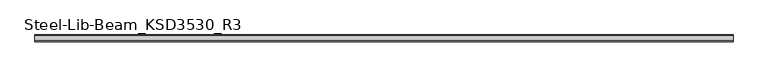
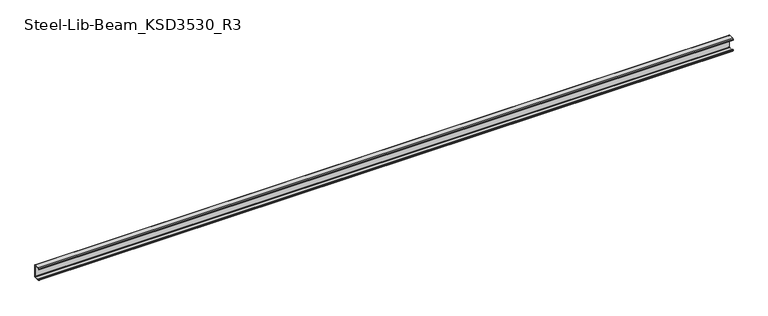
"""IFC4 building model written with IfcOpenShell, lengths in millimetres: beam geometry, Steel-Lib-Beam_KSD3530_R3 : BMS291_C-150×75x20x4.5."""

from ifc_helpers import new_model, si_unit, point, frame, frame_2d, origin, place, context, project, spatial, polyline, circle_curve, trimmed, segment, composite_curve, outline, extrude, source, transform, mapped, element, save


def steel_lib_beam_ksd3530_r3_927b0633(model_context):
    return source(origin(), model_context, "Body", "SweptSolid", [
        extrude(outline(composite_curve([segment(trimmed(circle_curve(frame_2d((-41.0, 66.0)), 9.0), [point((-50.0, 66.0))], [point((-41.0, 75.0))], False, "CARTESIAN"), True, "CONTINUOUS"), segment(polyline([(-41.0, 75.0), (16.0, 75.0)]), True, "CONTINUOUS"), segment(trimmed(circle_curve(frame_2d((16.0, 66.0)), 9.0), [point((16.0, 75.0))], [point((25.0, 66.0))], False, "CARTESIAN"), True, "CONTINUOUS"), segment(polyline([(25.0, 66.0), (25.0, -66.0)]), True, "CONTINUOUS"), segment(trimmed(circle_curve(frame_2d((16.0, -66.0)), 9.0), [point((25.0, -66.0))], [point((16.0, -75.0))], False, "CARTESIAN"), True, "CONTINUOUS"), segment(polyline([(16.0, -75.0), (-41.0, -75.0)]), True, "CONTINUOUS"), segment(trimmed(circle_curve(frame_2d((-41.0, -66.0)), 9.0), [point((-41.0, -75.0))], [point((-50.0, -66.0))], False, "CARTESIAN"), True, "CONTINUOUS"), segment(polyline([(-50.0, -66.0), (-50.0, -55.0), (-45.5, -55.0), (-45.5, -66.0)]), True, "CONTINUOUS"), segment(trimmed(circle_curve(frame_2d((-41.0, -66.0)), 4.5), [point((-45.5, -66.0))], [point((-41.0, -70.5))], True, "CARTESIAN"), True, "CONTINUOUS"), segment(polyline([(-41.0, -70.5), (16.0, -70.5)]), True, "CONTINUOUS"), segment(trimmed(circle_curve(frame_2d((16.0, -66.0)), 4.5), [point((16.0, -70.5))], [point((20.5, -66.0))], True, "CARTESIAN"), True, "CONTINUOUS"), segment(polyline([(20.5, -66.0), (20.5, 66.0)]), True, "CONTINUOUS"), segment(trimmed(circle_curve(frame_2d((16.0, 66.0)), 4.5), [point((20.5, 66.0))], [point((16.0, 70.5))], True, "CARTESIAN"), True, "CONTINUOUS"), segment(polyline([(16.0, 70.5), (-41.0, 70.5)]), True, "CONTINUOUS"), segment(trimmed(circle_curve(frame_2d((-41.0, 66.0)), 4.5), [point((-41.0, 70.5))], [point((-45.5, 66.0))], True, "CARTESIAN"), True, "CONTINUOUS"), segment(polyline([(-45.5, 66.0), (-45.5, 55.0), (-50.0, 55.0), (-50.0, 66.0)]), True, "CONTINUOUS")], self_intersect=False)), frame((-3897.5, 0.0, 0.0), z_axis=(1.0, 0.0, 0.0), x_axis=(0.0, 1.0, 0.0)), (0.0, 0.0, 1.0), 7795.0),
    ])


if __name__ == "__main__":
    model = new_model("IFC4")
    model_context = context("Model", 3, world=origin())
    ifc_project = project(units=[si_unit("LENGTHUNIT", "METRE", prefix="MILLI")], contexts=[model_context])
    site = spatial("IfcSite", under=ifc_project)
    building = spatial("IfcBuilding", under=site)
    placement = place(None, origin())
    steel_lib_beam_ksd3530_r3_shape = steel_lib_beam_ksd3530_r3_927b0633(model_context)
    element("IfcBeam", 1, ObjectType="Steel-Lib-Beam_KSD3530_R3 : BMS291_C-150×75x20x4.5", at=placement, inside=building, context=model_context, shape_type="MappedRepresentation", body=[
        mapped(steel_lib_beam_ksd3530_r3_shape, transform((0.0, 0.0, 0.0), x_axis=(1.0, 0.0, 0.0), y_axis=(0.0, 1.0, 0.0), z_axis=(0.0, 0.0, 1.0))),
    ])
    save(model, "model.ifc")

# Revit data of these elements
# Type "Steel-Lib-Beam_KSD3530_R3 : BMS291_C-150×75x20x4.5"
#   Keynote = "C-150×75x20x4.5"
#   SteelWeight = "Light"
#   x = 0.0250 m
#   t1 = 0.0090 m
#   t = 0.0045 m
#   Surface Area = 0.629834 m²/m
#   Section Area = 13.9688 cm²
#   Mass per Unit Length = 10.9655 kg/m
#   C = 0.0200 m
#   A = 0.0750 m
#   Length [instance default] = 1.5000 m
#   H = 0.1500 m
#   hec_material4 [instance default] = none
#   hec_material3 [instance default] = none
#   hec_material2 [instance default] = none
#   hec_material1 [instance default] = none
#   Structural Material [instance default] = Metal - Steel - Light Gauge
#   Assembly Code = ""
# Element 1 (IfcBeam, "Steel-Lib-Beam_KSD3530_R3 : BMS291_C-150×75x20x4.5")
#   Structural Material = none
# Materials
#   "Metal - Steel - Light Gauge": class "Metal", colour RGB 247 247 247, transparency 0
